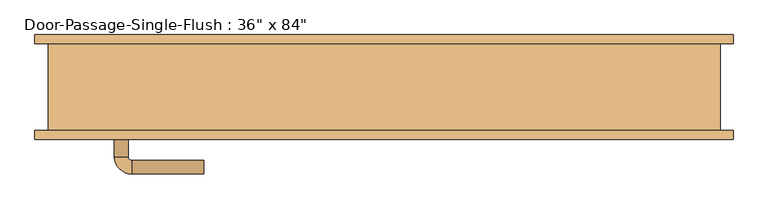
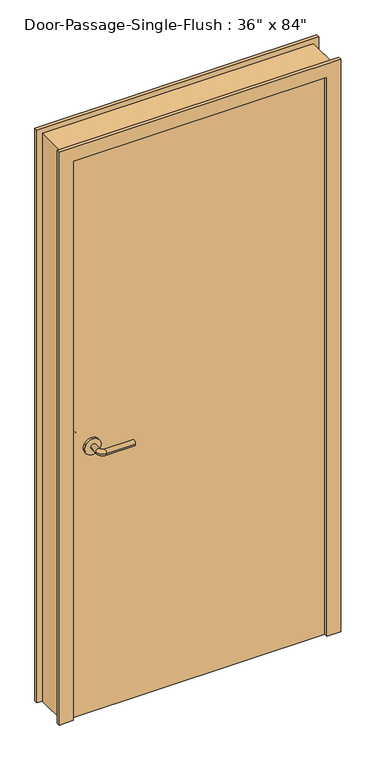
"""IFC4 building model written with IfcOpenShell, lengths in millimetres: door geometry."""

from ifc_helpers import new_model, si_unit, point, frame, frame_2d, origin, origin_with_axes, place, context, project, spatial, polyline, circle_curve, ellipse_curve, trimmed, segment, composite_curve, outline, extrude, faceted_brep, source, transform, mapped, element, save
from ifc_brep_helpers import plane_surface, cylinder_surface, revolved_surface, advanced_brep


def door_efefef0e(model_context):
    return source(origin(), model_context, "Body", "SolidModel", [
        advanced_brep(
        [(-392.190625, -17.4, 1016.0), (-372.190625, -17.4, 1016.0), (-392.190625, 12.6, 1016.0), (-372.190625, 12.6, 1016.0), (-367.190625, 17.6, 1016.0), (-367.190625, 37.6, 1016.0), (-262.190625, 37.6, 1016.0), (-262.190625, 17.6, 1016.0)],
        [
            (0, 1, circle_curve(frame((-382.190625, -17.4, 1016.0), z_axis=(0.0, -1.0, 0.0), x_axis=(1.0, 0.0, 0.0)), 10.0)),
            (1, 0, circle_curve(frame((-382.190625, -17.4, 1016.0), z_axis=(0.0, -1.0, 0.0), x_axis=(1.0, 0.0, 0.0)), 10.0)),
            (0, 2),
            (2, 3, circle_curve(frame((-382.190625, 12.6, 1016.0), z_axis=(0.0, -1.0, 0.0), x_axis=(1.0, 0.0, 0.0)), 10.0)),
            (3, 1),
            (3, 2, circle_curve(frame((-382.190625, 12.6, 1016.0), z_axis=(0.0, -1.0, 0.0), x_axis=(1.0, 0.0, 0.0)), 10.0)),
            (4, 3, circle_curve(frame((-367.190625, 12.6, 1016.0), z_axis=(0.0, 0.0, 1.0), x_axis=(-1.0, 0.0, 0.0)), 5.0)),
            (2, 5, circle_curve(frame((-367.190625, 12.6, 1016.0), z_axis=(0.0, 0.0, -1.0), x_axis=(-1.0, 0.0, 0.0)), 25.0)),
            (5, 4, circle_curve(frame((-367.190625, 27.6, 1016.0), z_axis=(-1.0, 0.0, 0.0), x_axis=(0.0, -1.0, 0.0)), 10.0)),
            (4, 5, circle_curve(frame((-367.190625, 27.6, 1016.0), z_axis=(-1.0, 0.0, 0.0), x_axis=(0.0, -1.0, 0.0)), 10.0)),
            (6, 7, circle_curve(frame((-262.190625, 27.6, 1016.0), z_axis=(1.0, 0.0, 0.0), x_axis=(0.0, -1.0, 0.0)), 10.0)),
            (7, 6, circle_curve(frame((-262.190625, 27.6, 1016.0), z_axis=(1.0, 0.0, 0.0), x_axis=(0.0, -1.0, 0.0)), 10.0)),
            (5, 6),
            (7, 4),
        ],
        [
            plane_surface(frame((-382.190625, -17.4, 1016.0), z_axis=(0.0, -1.0, 0.0), x_axis=(0.0, 0.0, 1.0))),
            cylinder_surface(frame((-382.190625, -17.4, 1016.0), z_axis=(0.0, -1.0, 0.0), x_axis=(1.0, 0.0, 0.0)), 10.0),
            revolved_surface(trimmed(ellipse_curve(frame((-382.190625, 12.6, 1016.0), z_axis=(0.0, -1.0, 0.0), x_axis=(1.0, 0.0, 0.0)), 10.0, 10.0), [point((-392.190625, 12.6, 1016.0))], [point((-372.190625, 12.6, 1016.0))], True, "CARTESIAN"), (-367.190625, 12.6, 1016.0), (0.0, 0.0, -1.0)),
            revolved_surface(trimmed(ellipse_curve(frame((-382.190625, 12.6, 1016.0), z_axis=(0.0, -1.0, 0.0), x_axis=(1.0, 0.0, 0.0)), 10.0, 10.0), [point((-372.190625, 12.6, 1016.0))], [point((-392.190625, 12.6, 1016.0))], True, "CARTESIAN"), (-367.190625, 12.6, 1016.0), (0.0, 0.0, -1.0)),
            plane_surface(frame((-262.190625, 27.6, 1016.0), z_axis=(1.0, 0.0, 0.0), x_axis=(0.0, 0.0, 1.0))),
            cylinder_surface(frame((-367.190625, 27.6, 1016.0), z_axis=(-1.0, 0.0, 0.0), x_axis=(0.0, -1.0, 0.0)), 10.0),
        ],
        [
            (0, [[1, 2]]),
            (1, [[-1, 3, 4, 5]]),
            (1, [[-2, -5, 6, -3]]),
            (2, [[7, -4, 8, 9]]),
            (3, [[-8, -6, -7, 10]]),
            (4, [[11, 12]]),
            (5, [[-9, 13, -12, 14]]),
            (5, [[-10, -14, -11, -13]]),
        ],
    ),
        extrude(outline(composite_curve([segment(trimmed(circle_curve(frame_2d((1016.0, -384.690625)), 30.0), [point((1016.0, -414.690625))], [point((1016.0, -354.690625))], False, "CARTESIAN"), True, "CONTINUOUS"), segment(trimmed(circle_curve(frame_2d((1016.0, -384.690625)), 30.0), [point((1016.0, -354.690625))], [point((1016.0, -414.690625))], False, "CARTESIAN"), True, "CONTINUOUS")], self_intersect=False)), frame((0.0, -25.4, 0.0), z_axis=(0.0, 1.0, 0.0), x_axis=(0.0, 0.0, 1.0)), (0.0, 0.0, 1.0), 8.0),
        advanced_brep(
        [(-392.190625, -77.85, 1016.0), (-372.190625, -77.85, 1016.0), (-372.190625, -107.85, 1016.0), (-392.190625, -107.85, 1016.0), (-367.190625, -112.85, 1016.0), (-367.190625, -132.85, 1016.0), (-262.190625, -132.85, 1016.0), (-262.190625, -112.85, 1016.0)],
        [
            (0, 1, circle_curve(frame((-382.190625, -77.85, 1016.0), z_axis=(0.0, 1.0, 0.0), x_axis=(1.0, 0.0, 0.0)), 10.0)),
            (1, 0, circle_curve(frame((-382.190625, -77.85, 1016.0), z_axis=(0.0, 1.0, 0.0), x_axis=(1.0, 0.0, 0.0)), 10.0)),
            (1, 2),
            (2, 3, circle_curve(frame((-382.190625, -107.85, 1016.0), z_axis=(0.0, 1.0, 0.0), x_axis=(1.0, 0.0, 0.0)), 10.0)),
            (3, 0),
            (3, 2, circle_curve(frame((-382.190625, -107.85, 1016.0), z_axis=(0.0, 1.0, 0.0), x_axis=(1.0, 0.0, 0.0)), 10.0)),
            (4, 5, circle_curve(frame((-367.190625, -122.85, 1016.0), z_axis=(-1.0, 0.0, 0.0), x_axis=(0.0, 1.0, 0.0)), 10.0)),
            (5, 3, circle_curve(frame((-367.190625, -107.85, 1016.0), z_axis=(0.0, 0.0, -1.0), x_axis=(-1.0, 0.0, 0.0)), 25.0)),
            (2, 4, circle_curve(frame((-367.190625, -107.85, 1016.0), z_axis=(0.0, 0.0, 1.0), x_axis=(-1.0, 0.0, 0.0)), 5.0)),
            (5, 4, circle_curve(frame((-367.190625, -122.85, 1016.0), z_axis=(-1.0, 0.0, 0.0), x_axis=(0.0, 1.0, 0.0)), 10.0)),
            (6, 7, circle_curve(frame((-262.190625, -122.85, 1016.0), z_axis=(1.0, 0.0, 0.0), x_axis=(0.0, 1.0, 0.0)), 10.0)),
            (7, 6, circle_curve(frame((-262.190625, -122.85, 1016.0), z_axis=(1.0, 0.0, 0.0), x_axis=(0.0, 1.0, 0.0)), 10.0)),
            (4, 7),
            (6, 5),
        ],
        [
            plane_surface(frame((-382.190625, -77.85, 1016.0), z_axis=(0.0, 1.0, 0.0), x_axis=(0.0, 0.0, 1.0))),
            cylinder_surface(frame((-382.190625, -77.85, 1016.0), z_axis=(0.0, 1.0, 0.0), x_axis=(1.0, 0.0, 0.0)), 10.0),
            revolved_surface(trimmed(ellipse_curve(frame((-382.190625, -107.85, 1016.0), z_axis=(0.0, -1.0, 0.0), x_axis=(1.0, 0.0, 0.0)), 10.0, 10.0), [point((-392.190625, -107.85, 1016.0))], [point((-372.190625, -107.85, 1016.0))], True, "CARTESIAN"), (-367.190625, -107.85, 1016.0), (0.0, 0.0, -1.0)),
            revolved_surface(trimmed(ellipse_curve(frame((-382.190625, -107.85, 1016.0), z_axis=(0.0, -1.0, 0.0), x_axis=(1.0, 0.0, 0.0)), 10.0, 10.0), [point((-372.190625, -107.85, 1016.0))], [point((-392.190625, -107.85, 1016.0))], True, "CARTESIAN"), (-367.190625, -107.85, 1016.0), (0.0, 0.0, -1.0)),
            plane_surface(frame((-262.190625, -122.85, 1016.0), z_axis=(1.0, 0.0, 0.0), x_axis=(0.0, 0.0, 1.0))),
            cylinder_surface(frame((-367.190625, -122.85, 1016.0), z_axis=(-1.0, 0.0, 0.0), x_axis=(0.0, 1.0, 0.0)), 10.0),
        ],
        [
            (0, [[1, 2]]),
            (1, [[3, 4, 5, -2]]),
            (1, [[-5, 6, -3, -1]]),
            (2, [[7, 8, -4, 9]]),
            (3, [[10, -9, -6, -8]]),
            (4, [[11, 12]]),
            (5, [[13, -11, 14, -7]]),
            (5, [[-14, -12, -13, -10]]),
        ],
    ),
        extrude(outline(composite_curve([segment(trimmed(circle_curve(frame_2d((1016.0, -384.690625)), 30.0), [point((1016.0, -414.690625))], [point((1016.0, -354.690625))], False, "CARTESIAN"), True, "CONTINUOUS"), segment(trimmed(circle_curve(frame_2d((1016.0, -384.690625)), 30.0), [point((1016.0, -354.690625))], [point((1016.0, -414.690625))], False, "CARTESIAN"), True, "CONTINUOUS")], self_intersect=False)), frame((0.0, -77.85, 0.0), z_axis=(0.0, 1.0, 0.0), x_axis=(0.0, 0.0, 1.0)), (0.0, 0.0, 1.0), 8.0),
        faceted_brep([(457.2, -82.55, 0.0), (457.2, -20.6375, 0.0), (441.325, -20.6375, 0.0), (441.325, 17.4625, 0.0), (457.2, 17.4625, 0.0), (457.2, 69.85, 0.0), (508.0, 69.85, 0.0), (508.0, 57.15, 0.0), (488.95, 57.15, 0.0), (488.95, -69.85, 0.0), (508.0, -69.85, 0.0), (508.0, -82.55, 0.0), (508.0, -82.55, 2184.4), (-508.0, -82.55, 2184.4), (-508.0, -82.55, 0.0), (-457.2, -82.55, 0.0), (-457.2, -82.55, 2133.6), (457.2, -82.55, 2133.6), (508.0, -69.85, 2184.4), (488.95, -69.85, 2165.35), (-488.95, -69.85, 2165.35), (-488.95, -69.85, 0.0), (-508.0, -69.85, 0.0), (-508.0, -69.85, 2184.4), (488.95, 57.15, 2165.35), (508.0, 57.15, 2184.4), (-508.0, 57.15, 2184.4), (-508.0, 57.15, 0.0), (-488.95, 57.15, 0.0), (-488.95, 57.15, 2165.35), (508.0, 69.85, 2184.4), (457.2, 69.85, 2133.6), (-457.2, 69.85, 2133.6), (-457.2, 69.85, 0.0), (-508.0, 69.85, 0.0), (-508.0, 69.85, 2184.4), (457.2, 17.4625, 2133.6), (441.325, 17.4625, 2117.725), (-441.325, 17.4625, 2117.725), (-441.325, 17.4625, 0.0), (-457.2, 17.4625, 0.0), (-457.2, 17.4625, 2133.6), (441.325, -20.6375, 2117.725), (457.2, -20.6375, 2133.6), (-457.2, -20.6375, 2133.6), (-457.2, -20.6375, 0.0), (-441.325, -20.6375, 0.0), (-441.325, -20.6375, 2117.725)], [[[0, 1, 2, 3, 4, 5, 6, 7, 8, 9, 10, 11]], [[11, 12, 13, 14, 15, 16, 17, 0]], [[10, 18, 12, 11]], [[9, 19, 20, 21, 22, 23, 18, 10]], [[8, 24, 19, 9]], [[7, 25, 26, 27, 28, 29, 24, 8]], [[6, 30, 25, 7]], [[5, 31, 32, 33, 34, 35, 30, 6]], [[4, 36, 31, 5]], [[3, 37, 38, 39, 40, 41, 36, 4]], [[2, 42, 37, 3]], [[1, 43, 44, 45, 46, 47, 42, 2]], [[0, 17, 43, 1]], [[18, 23, 13, 12]], [[24, 29, 20, 19]], [[30, 35, 26, 25]], [[36, 41, 32, 31]], [[42, 47, 38, 37]], [[17, 16, 44, 43]], [[15, 14, 22, 21, 28, 27, 34, 33, 40, 39, 46, 45]], [[23, 22, 14, 13]], [[29, 28, 21, 20]], [[35, 34, 27, 26]], [[41, 40, 33, 32]], [[47, 46, 39, 38]], [[16, 15, 45, 44]]]),
        extrude(outline(polyline([(457.2, -25.4), (457.2, -69.85), (-457.2, -69.85), (-457.2, -25.4), (457.2, -25.4)])), origin_with_axes(), (0.0, 0.0, 1.0), 2133.6),
    ])


if __name__ == "__main__":
    model = new_model("IFC4")
    model_context = context("Model", 3, world=origin())
    ifc_project = project(units=[si_unit("LENGTHUNIT", "METRE", prefix="MILLI")], contexts=[model_context])
    site = spatial("IfcSite", under=ifc_project)
    building = spatial("IfcBuilding", under=site)
    placement = place(None, origin())
    door_shape = door_efefef0e(model_context)
    element("IfcDoor", 1, ObjectType="Door-Passage-Single-Flush : 36\" x 84\"", at=placement, inside=building, context=model_context, shape_type="MappedRepresentation", body=[
        mapped(door_shape, transform((0.0, 0.0, 0.0), x_axis=(1.0, 0.0, 0.0), y_axis=(0.0, 1.0, 0.0), z_axis=(0.0, 0.0, 1.0))),
    ])
    save(model, "model.ifc")

# Revit data of these elements
# Type "Door-Passage-Single-Flush : 36\" x 84\""
#   Type Mark = "19"
#   Fire Rating = "--"
#   Assembly Code = "B2030200"
#   Analytic Construction = "Wooden"
#   Thickness = 0' - 1 3/4"
#   Thermal Resistance (R) = 2.5876 (h·ft²·°F)/BTU
#   Swing Angle [instance default] = 90.00°
#   Strike Height = 3' - 4"
#   Rough Width [instance default] = 3' - 4"
#   Rough Height [instance default] = 7' - 4"
#   MF Opening Height [instance default] = 0' - 4"
#   MF Opening Width [instance default] = 0' - 4"
#   Inset Calculate [instance default] = 0' - 4"
#   Masonry Inset [instance default] = 0' - 1"
#   Height = 7' - 0"
#   Width = 3' - 0"
#   Heat Transfer Coefficient (U) = 0.3865 BTU/(h·ft²·°F)
#   Masonry Frame Depth = 0' - 5 3/4"
#   Masonry Frame [instance default] = yes
#   Function = 1
#   Dry Wall Frame [instance default] = no
#   Panel Material = Wood - Birch
#   Frame Material = Metal - Paint Finish - Grey
#   Door Handle Material = Aluminum
#   Visual Light Transmittance = 0
#   Solar Heat Gain Coefficient = 0
#   Wall Closure = (empty or 0)
# Element 1 (IfcDoor, "Door-Passage-Single-Flush : 36\" x 84\"")
#   Rough Width = 3' - 2 1/2"
#   Rough Height = 7' - 1 1/4"
#   MF Opening Height = 0' - 1 1/4"
#   MF Opening Width = 0' - 2 1/2"
#   Inset Calculate = 0' - 3"
#   Masonry Frame = no
#   Dry Wall Frame = yes
#   Materials on its faces: "Metal - Paint Finish - Grey", "Aluminum", "Wood - Birch"
# Materials
#   "Wood - Birch": class "Wood", colour RGB 166 116 52, transparency 0, Cost = 0
#   "Metal - Paint Finish - Grey": class "Paint", colour RGB 104 104 104, transparency 0, Cost = 0
#   "Aluminum": class "Metal", colour RGB 247 247 247, transparency 0, Description = "Aluminum 6061", Cost = 0
